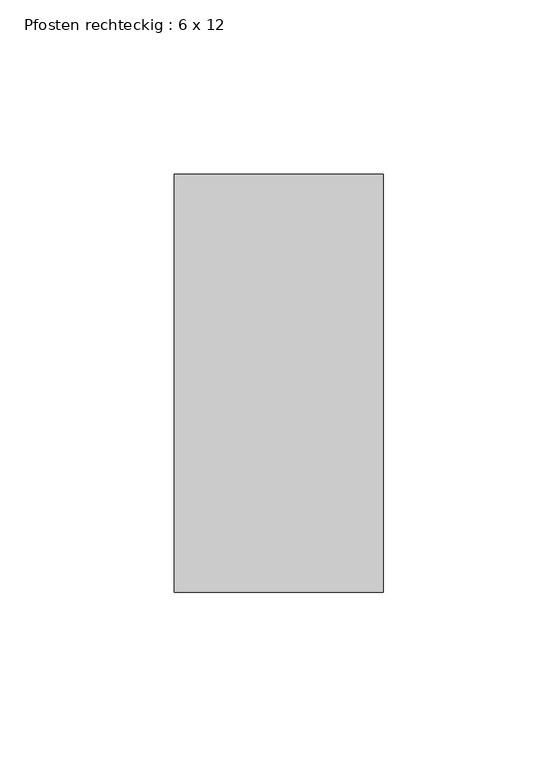
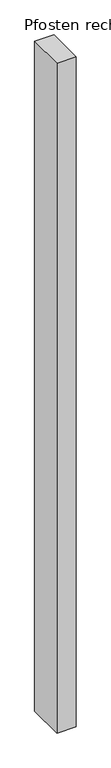
"""IFC4 building model written with IfcOpenShell, lengths in millimetres: member geometry, Pfosten rechteckig : 6 x 12."""

from ifc_helpers import new_model, si_unit, frame, origin, place, context, project, spatial, polyline, outline, extrude, source, transform, mapped, element, save


def pfosten_rechteckig_6_x_12_07b093b4(model_context):
    return source(origin(), model_context, "Body", "SweptSolid", [
        extrude(outline(polyline([(0.0, 60.0), (0.0, -60.0), (-60.0, -60.0), (-60.0, 60.0), (0.0, 60.0)])), frame((0.0, 0.0, -2220.0), z_axis=(0.0, 0.0, 1.0), x_axis=(1.0, 0.0, 0.0)), (0.0, 0.0, 1.0), 2220.0),
    ])


if __name__ == "__main__":
    model = new_model("IFC4")
    model_context = context("Model", 3, world=origin())
    ifc_project = project(units=[si_unit("LENGTHUNIT", "METRE", prefix="MILLI")], contexts=[model_context])
    site = spatial("IfcSite", under=ifc_project)
    building = spatial("IfcBuilding", under=site)
    placement = place(None, origin())
    pfosten_rechteckig_6_x_12_shape = pfosten_rechteckig_6_x_12_07b093b4(model_context)
    element("IfcMember", 1, ObjectType="Pfosten rechteckig : 6 x 12", at=placement, inside=building, context=model_context, shape_type="MappedRepresentation", body=[
        mapped(pfosten_rechteckig_6_x_12_shape, transform((0.0, 0.0, 0.0), x_axis=(1.0, 0.0, 0.0), y_axis=(0.0, 1.0, 0.0), z_axis=(0.0, 0.0, 1.0))),
    ])
    save(model, "model.ifc")

# Revit data of these elements
# Project information
#   Projektausgabedatum = "Projekt Datum"
#   Projektstatus = "Projektstatus"
#   Kundenname = "Bauherr"
#   Projektadresse = "Projektadresse"
#   Projektname = "Projektname"
#   Projektnummer = "Projektnummer"
#   Verfasser Firma 1 = "Firma 1"
#   Verfasser Firma 2 = "Firma 2"
#   Verfasser PLZ Ort = "PLZ Ort"
#   Verfasser Strasse = "Strasse"
#   Verfasser Telefon = "Telefon"
#   Verfasser Telefax = "Telefax"
#   Verfasser eMail = "E-Mail"
# Type "Pfosten rechteckig : 6 x 12"
#   built-in parameter 1007304 = 0.393701 (stored number, unit not read)
#   built-in parameter 1007301 = 0.0984252 (stored number, unit not read)
#   built-in parameter 1007300 = 0.0984252 (stored number, unit not read)
# Element 1 (IfcMember, "Pfosten rechteckig : 6 x 12")
#   Materials on its faces: "Metall - verzinkt"
# Materials
#   "Metall - verzinkt": class "Allgemeines", colour RGB 200 200 200, transparency 0, Cost = 0
